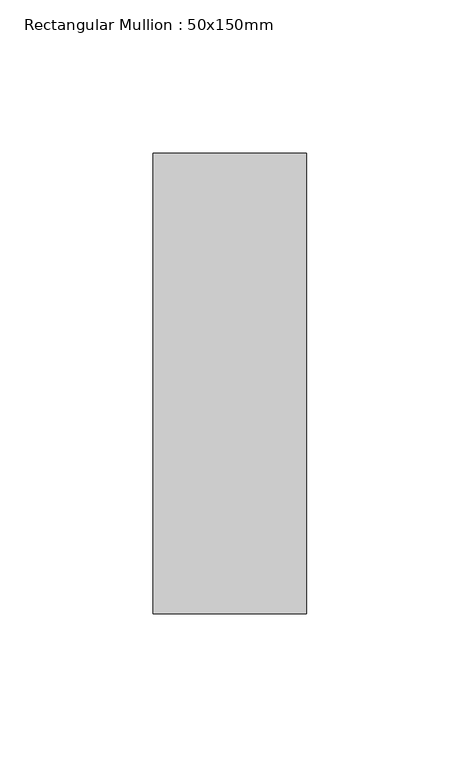
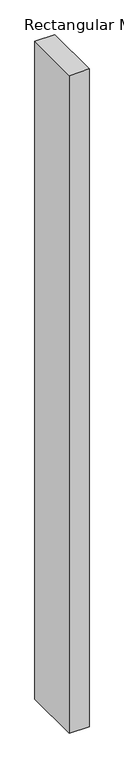
"""IFC4 building model written with IfcOpenShell, lengths in millimetres: member geometry, Rectangular Mullion : 50x150mm."""

from ifc_helpers import new_model, si_unit, frame, origin, place, context, project, spatial, polyline, outline, extrude, source, transform, mapped, element, save


def rectangular_mullion_50x150mm_4f45a924(model_context):
    return source(origin(), model_context, "Body", "SweptSolid", [
        extrude(outline(polyline([(0.0, 75.0), (0.0, -75.0), (-50.0, -75.0), (-50.0, 75.0), (0.0, 75.0)])), frame((0.0, 0.0, -1755.0000003), z_axis=(0.0, 0.0, 1.0), x_axis=(1.0, 0.0, 0.0)), (0.0, 0.0, 1.0), 1755.0000003),
    ])


if __name__ == "__main__":
    model = new_model("IFC4")
    model_context = context("Model", 3, world=origin())
    ifc_project = project(units=[si_unit("LENGTHUNIT", "METRE", prefix="MILLI")], contexts=[model_context])
    site = spatial("IfcSite", under=ifc_project)
    building = spatial("IfcBuilding", under=site)
    placement = place(None, origin())
    rectangular_mullion_50x150mm_shape = rectangular_mullion_50x150mm_4f45a924(model_context)
    element("IfcMember", 1, ObjectType="Rectangular Mullion : 50x150mm", at=placement, inside=building, context=model_context, shape_type="MappedRepresentation", body=[
        mapped(rectangular_mullion_50x150mm_shape, transform((0.0, 0.0, 0.0), x_axis=(1.0, 0.0, 0.0), y_axis=(0.0, 1.0, 0.0), z_axis=(0.0, 0.0, 1.0))),
    ])
    save(model, "model.ifc")

# Revit data of these elements
# Type "Rectangular Mullion : 50x150mm"
#   Keynote = "H11"
#   built-in parameter 1007304 = 0.492126 (stored number, unit not read)
#   built-in parameter 1007301 = 0.082021 (stored number, unit not read)
#   built-in parameter 1007300 = 0.082021 (stored number, unit not read)
# Element 1 (IfcMember, "Rectangular Mullion : 50x150mm")
#   Materials on its faces: "Aluminium"
# Materials
#   "Aluminium": class "Metal", colour RGB 247 247 247, transparency 0, Description = "Aluminium 6061", Cost = 0
